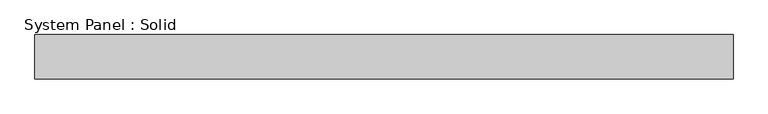
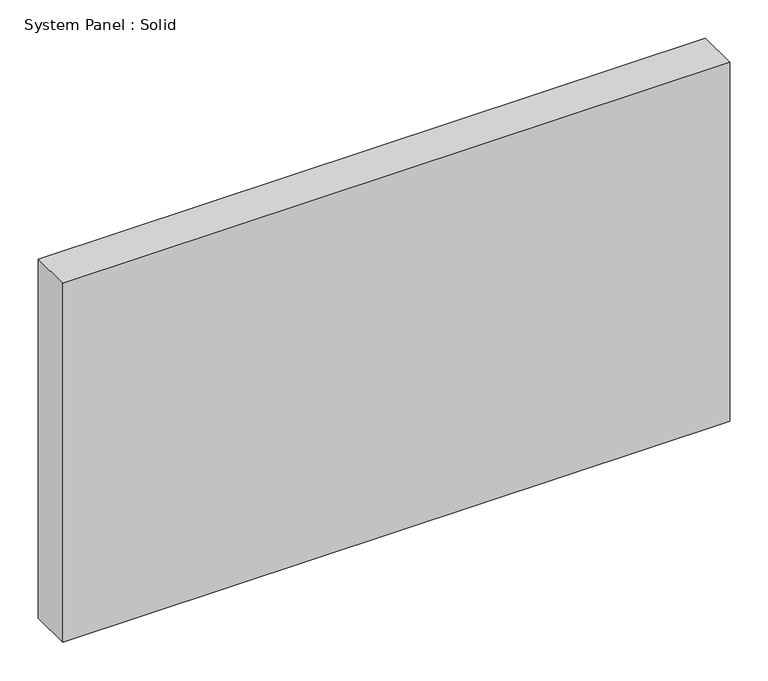
"""IFC4 building model written with IfcOpenShell, lengths in millimetres: plate geometry, System Panel : Solid."""

from ifc_helpers import new_model, si_unit, origin, origin_with_axes, place, context, project, spatial, polyline, outline, extrude, source, transform, mapped, element, save


def system_panel_solid_1ca27012(model_context):
    return source(origin(), model_context, "Body", "SweptSolid", [
        extrude(outline(polyline([(502.4643964, -19.05), (-502.4643964, -19.05), (-502.4643964, 44.45), (502.4643964, 44.45), (502.4643964, -19.05)])), origin_with_axes(), (0.0, 0.0, 1.0), 571.5),
    ])


if __name__ == "__main__":
    model = new_model("IFC4")
    model_context = context("Model", 3, world=origin())
    ifc_project = project(units=[si_unit("LENGTHUNIT", "METRE", prefix="MILLI")], contexts=[model_context])
    site = spatial("IfcSite", under=ifc_project)
    building = spatial("IfcBuilding", under=site)
    placement = place(None, origin())
    system_panel_solid_shape = system_panel_solid_1ca27012(model_context)
    element("IfcPlate", 1, ObjectType="System Panel : Solid", at=placement, inside=building, context=model_context, shape_type="MappedRepresentation", body=[
        mapped(system_panel_solid_shape, transform((0.0, 0.0, 0.0), x_axis=(1.0, 0.0, 0.0), y_axis=(0.0, 1.0, 0.0), z_axis=(0.0, 0.0, 1.0))),
    ])
    save(model, "model.ifc")

# Revit data of these elements
# Element 1 (IfcPlate, "System Panel : Solid")
#   Materials on its faces: "Default"
# Materials
#   "Default": class "Miscellaneous", colour RGB 127 127 127, transparency 0
